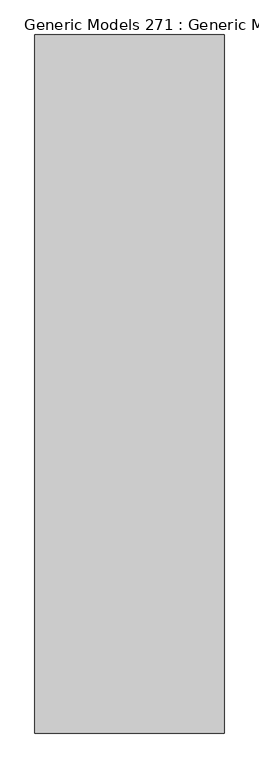
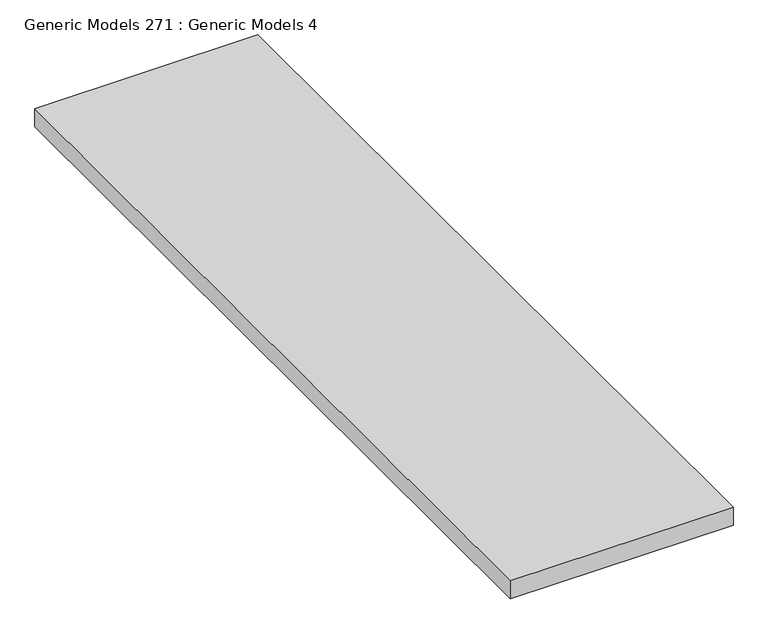
"""IFC4 building model written with IfcOpenShell, lengths in millimetres: proxy geometry, Generic Models 271 : Generic Models 4."""

from ifc_helpers import new_model, si_unit, frame, origin, place, context, project, spatial, polyline, outline, extrude, source, transform, mapped, element, save


def generic_models_271_generic_models_4_3a861936(model_context):
    return source(origin(), model_context, "Body", "SweptSolid", [
        extrude(outline(polyline([(-6629.5736296, -5493.3230338), (-10028.1472239, -5493.3230338), (-10028.1472239, 7054.2769662), (-6629.5736296, 7054.2769662), (-6629.5736296, -5493.3230338)])), frame((0.0, 0.0, 122511.1484874), z_axis=(0.0, 0.0, 1.0), x_axis=(1.0, 0.0, 0.0)), (0.0, 0.0, 1.0), 292.1),
    ])


if __name__ == "__main__":
    model = new_model("IFC4")
    model_context = context("Model", 3, world=origin())
    ifc_project = project(units=[si_unit("LENGTHUNIT", "METRE", prefix="MILLI")], contexts=[model_context])
    site = spatial("IfcSite", under=ifc_project)
    building = spatial("IfcBuilding", under=site)
    placement = place(None, origin())
    generic_models_271_generic_models_4_shape = generic_models_271_generic_models_4_3a861936(model_context)
    element("IfcBuildingElementProxy", 1, Name="Generic Models 271 : Generic Models 4", ObjectType="Generic Models 271 : Generic Models 4", at=placement, inside=building, context=model_context, shape_type="MappedRepresentation", body=[
        mapped(generic_models_271_generic_models_4_shape, transform((0.0, 0.0, 0.0), x_axis=(1.0, 0.0, 0.0), y_axis=(0.0, 1.0, 0.0), z_axis=(0.0, 0.0, 1.0))),
    ])
    save(model, "model.ifc")

# Revit data of these elements
# Element 1 (IfcBuildingElementProxy, "Generic Models 271 : Generic Models 4")
#   Materials on its faces: "_COMPACTED GRADE"
# Materials
#   "_COMPACTED GRADE": class "Generic", colour RGB 120 100 58, transparency 0, Cost = 0
